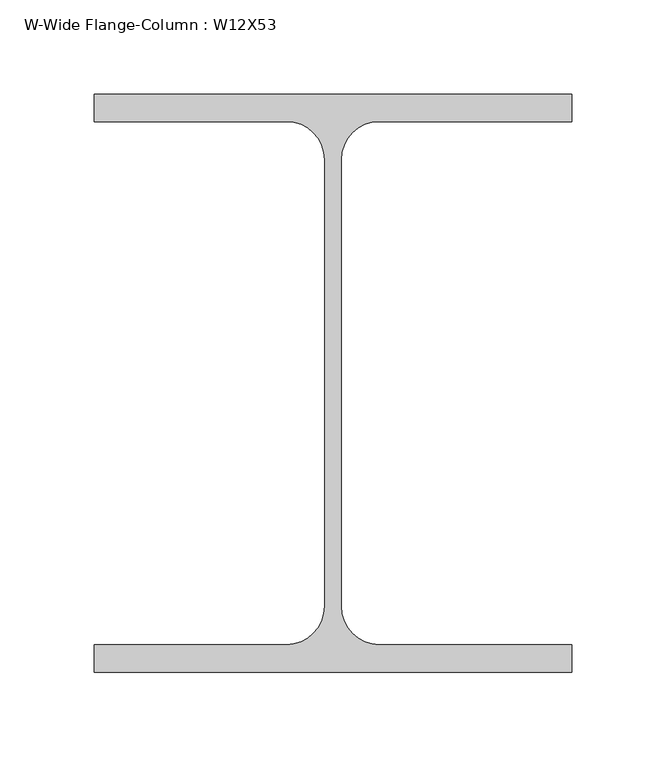
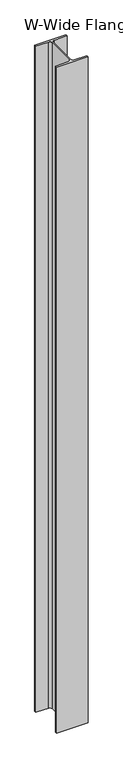
"""IFC4 building model written with IfcOpenShell, lengths in millimetres: column geometry, W-Wide Flange-Column : W12X53."""

from ifc_helpers import new_model, si_unit, point, frame, frame_2d, origin, place, context, project, spatial, polyline, circle_curve, trimmed, segment, composite_curve, outline, extrude, source, transform, mapped, element, save


def w_wide_flange_column_w12x53_a2bdef27(model_context):
    return source(origin(), model_context, "Body", "SweptSolid", [
        extrude(outline(composite_curve([segment(polyline([(127.0, 153.67), (127.0, 139.065), (24.7015, 139.065)]), True, "CONTINUOUS"), segment(trimmed(circle_curve(frame_2d((24.7015, 118.745)), 20.32), [point((24.7015, 139.065))], [point((4.3815, 118.745))], True, "CARTESIAN"), True, "CONTINUOUS"), segment(polyline([(4.3815, 118.745), (4.3815, -118.745)]), True, "CONTINUOUS"), segment(trimmed(circle_curve(frame_2d((24.7015, -118.745)), 20.32), [point((4.3815, -118.745))], [point((24.7015, -139.065))], True, "CARTESIAN"), True, "CONTINUOUS"), segment(polyline([(24.7015, -139.065), (127.0, -139.065), (127.0, -153.67), (-127.0, -153.67), (-127.0, -139.065), (-24.7015, -139.065)]), True, "CONTINUOUS"), segment(trimmed(circle_curve(frame_2d((-24.7015, -118.745)), 20.32), [point((-24.7015, -139.065))], [point((-4.3815, -118.745))], True, "CARTESIAN"), True, "CONTINUOUS"), segment(polyline([(-4.3815, -118.745), (-4.3815, 118.745)]), True, "CONTINUOUS"), segment(trimmed(circle_curve(frame_2d((-24.7015, 118.745)), 20.32), [point((-4.3815, 118.745))], [point((-24.7015, 139.065))], True, "CARTESIAN"), True, "CONTINUOUS"), segment(polyline([(-24.7015, 139.065), (-127.0, 139.065), (-127.0, 153.67), (127.0, 153.67)]), True, "CONTINUOUS")], self_intersect=False)), frame((0.0, 0.0, 23317.2), z_axis=(0.0, 0.0, 1.0), x_axis=(1.0, 0.0, 0.0)), (0.0, 0.0, 1.0), 5689.6),
    ])


if __name__ == "__main__":
    model = new_model("IFC4")
    model_context = context("Model", 3, world=origin())
    ifc_project = project(units=[si_unit("LENGTHUNIT", "METRE", prefix="MILLI")], contexts=[model_context])
    site = spatial("IfcSite", under=ifc_project)
    building = spatial("IfcBuilding", under=site)
    placement = place(None, origin())
    w_wide_flange_column_w12x53_shape = w_wide_flange_column_w12x53_a2bdef27(model_context)
    element("IfcColumn", 1, ObjectType="W-Wide Flange-Column : W12X53", at=placement, inside=building, context=model_context, shape_type="MappedRepresentation", body=[
        mapped(w_wide_flange_column_w12x53_shape, transform((0.0, 0.0, 0.0), x_axis=(1.0, 0.0, 0.0), y_axis=(0.0, 1.0, 0.0), z_axis=(0.0, 0.0, 1.0))),
    ])
    save(model, "model.ifc")

# Revit data of these elements
# Type "W-Wide Flange-Column : W12X53"
#   Assembly Code = "B10"
#   W = 53
#   bf = 0' - 10"
#   d = 1' - 0.1"
#   k = 0' - 1 3/8"
#   kr = 0' - 0.8"
#   tf = 0' - 0.575"
#   tw = 0' - 0.345"
#   A = 0.108333 SF
#   Structural Material [instance default] = Steel ASTM A992
# Element 1 (IfcColumn, "W-Wide Flange-Column : W12X53")
#   Materials on its faces: "Steel ASTM A992"
# Materials
#   "Steel ASTM A992": class "Metal", colour RGB 199 199 199, transparency 0, Description = "Structural steel 50ksi", Cost = 0
